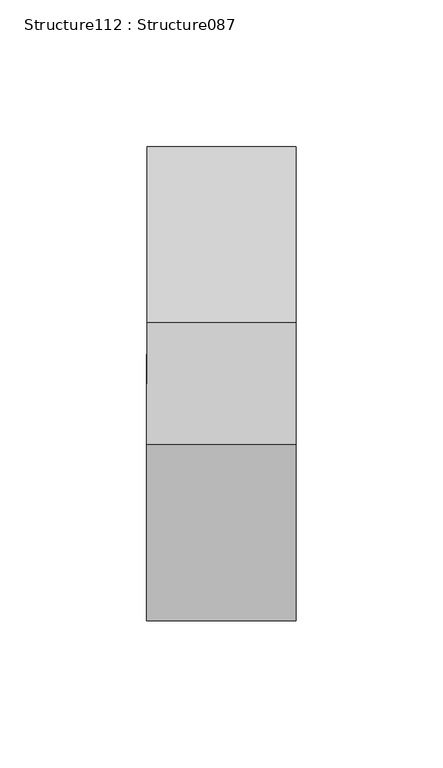
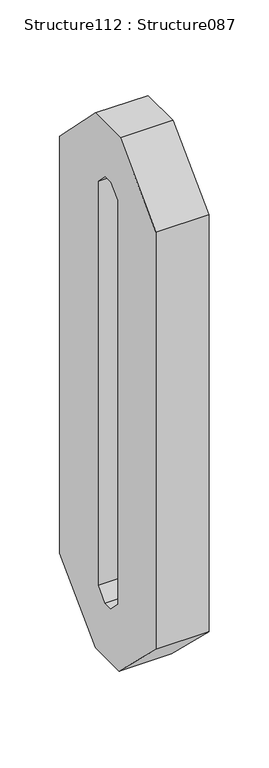
"""IFC4 building model written with IfcOpenShell, lengths in millimetres: proxy geometry, Structure112 : Structure087."""

import ifcopenshell
import ifcopenshell.guid

model = None  # the IFC model being written
_history = None  # IfcOwnerHistory: only IFC2X3 demands one
_inside = {}  # id of a spatial element -> (the spatial element, [elements in it])
_under = {}  # id of a project, library or spatial element -> (it, [spatial elements below it])
_declared = {}  # id of a project -> (the project, [libraries it declares])
_typed = {}  # id of a type object -> (the type object, [elements of that type])
_made_of = {}  # id of a material, layer set ... -> (it, [elements and type objects made of it])


def new_model(schema):
    """Start an empty IFC model of exactly this schema.

    Asked for "IFC4X3", IfcOpenShell would pick the latest addendum, in which some entities
    have other attributes; the version numbers below select the first issue.
    IFC2X3 requires an IfcOwnerHistory on every rooted entity: one is made here for all.
    """
    global model, _history
    if schema == "IFC4X3":
        model = ifcopenshell.file(schema_version=(4, 3, 0, 0))
    else:
        model = ifcopenshell.file(schema=schema)
    _inside.clear()
    _under.clear()
    _declared.clear()
    _typed.clear()
    _made_of.clear()
    _history = None
    if model.schema == "IFC2X3":
        org = make("IfcOrganization", Name="unknown")
        user = make(
            "IfcPersonAndOrganization",
            ThePerson=make("IfcPerson", FamilyName="unknown"),
            TheOrganization=org,
        )
        app = make(
            "IfcApplication",
            ApplicationDeveloper=org,
            Version="unknown",
            ApplicationFullName="unknown",
            ApplicationIdentifier="unknown",
        )
        _history = make(
            "IfcOwnerHistory",
            OwningUser=user,
            OwningApplication=app,
            ChangeAction="ADDED",
            CreationDate=0,
        )
    return model


def make(cls, **values):
    """One entity of the class cls with the attributes given. An attribute that is None is left unset."""
    return model.create_entity(
        cls, **{name: value for name, value in values.items() if value is not None}
    )


def rooted(cls, **values):
    """An entity with a GlobalId (a new one), such as an element, a storey or a relation."""
    return make(cls, GlobalId=ifcopenshell.guid.new(), OwnerHistory=_history, **values)


def si_unit(unit_type, name, prefix=None):
    """IfcSIUnit, for example si_unit("LENGTHUNIT", "METRE", prefix="MILLI")."""
    return make("IfcSIUnit", UnitType=unit_type, Prefix=prefix, Name=name)


def assignment(units):
    """IfcUnitAssignment: the units of a project."""
    return None if units is None else make("IfcUnitAssignment", Units=units)


def point(xyz):
    """IfcCartesianPoint."""
    return None if xyz is None else make("IfcCartesianPoint", Coordinates=xyz)


def direction(xyz):
    """IfcDirection."""
    return None if xyz is None else make("IfcDirection", DirectionRatios=xyz)


def frame(location, z_axis=None, x_axis=None):
    """IfcAxis2Placement3D, a coordinate frame: its origin and axes. An axis left out is left unset."""
    return make(
        "IfcAxis2Placement3D",
        Location=point(location),
        Axis=direction(z_axis),
        RefDirection=direction(x_axis),
    )


def origin():
    """The frame at (0, 0, 0) with its axes left unset."""
    return frame((0.0, 0.0, 0.0))


def place(relative_to, where):
    """IfcLocalPlacement: puts the frame where relative to a parent placement (None: the world)."""
    return make(
        "IfcLocalPlacement", PlacementRelTo=relative_to, RelativePlacement=where
    )


def context(
    kind, dimensions, precision=None, world=None, true_north=None, identifier=None
):
    """IfcGeometricRepresentationContext, for example the 3D "Model" context."""
    return make(
        "IfcGeometricRepresentationContext",
        ContextIdentifier=identifier,
        ContextType=kind,
        CoordinateSpaceDimension=dimensions,
        Precision=precision,
        WorldCoordinateSystem=world,
        TrueNorth=true_north,
    )


def project(units=None, contexts=None):
    """IfcProject with its units and contexts."""
    return rooted(
        "IfcProject",
        Name="project",
        RepresentationContexts=contexts,
        UnitsInContext=assignment(units),
    )


def spatial(cls, under=None, at=None, **own):
    """A site, building, storey or space (cls), placed at a placement, below another one or the project."""
    s = rooted(cls, ObjectPlacement=at, **own)
    if under is not None:
        _under.setdefault(under.id(), (under, []))[1].append(s)
    return s


def polyline(points):
    """IfcPolyline through the points."""
    return make("IfcPolyline", Points=[point(p) for p in points])


def outline(outer, holes=None, kind="AREA"):
    """IfcArbitraryClosedProfileDef: a profile drawn as a closed curve; with holes, ...WithVoids."""
    if holes is None:
        return make("IfcArbitraryClosedProfileDef", ProfileType=kind, OuterCurve=outer)
    return make(
        "IfcArbitraryProfileDefWithVoids",
        ProfileType=kind,
        OuterCurve=outer,
        InnerCurves=holes,
    )


def extrude(swept, where, along, depth):
    """IfcExtrudedAreaSolid: the profile swept, set in the frame where, extruded along a direction by depth."""
    return make(
        "IfcExtrudedAreaSolid",
        SweptArea=swept,
        Position=where,
        ExtrudedDirection=direction(along),
        Depth=depth,
    )


def shape(context_of_items, identifier, shape_type, items):
    """IfcShapeRepresentation: the items that make up one representation, for example the "Body"."""
    return make(
        "IfcShapeRepresentation",
        ContextOfItems=context_of_items,
        RepresentationIdentifier=identifier,
        RepresentationType=shape_type,
        Items=items,
    )


def source(mapping_origin, context_of_items, identifier, shape_type, items):
    """IfcRepresentationMap: a shape defined once, which mapped items show again and again."""
    return make(
        "IfcRepresentationMap",
        MappingOrigin=mapping_origin,
        MappedRepresentation=shape(context_of_items, identifier, shape_type, items),
    )


def transform(
    local_origin,
    x_axis=None,
    y_axis=None,
    z_axis=None,
    scale=None,
    scale2=None,
    scale3=None,
    uniform=True,
):
    """IfcCartesianTransformationOperator3D, or its non-uniform kind. x_axis, y_axis, z_axis: its Axis1, 2, 3."""
    if uniform:
        return make(
            "IfcCartesianTransformationOperator3D",
            Axis1=direction(x_axis),
            Axis2=direction(y_axis),
            LocalOrigin=point(local_origin),
            Scale=scale,
            Axis3=direction(z_axis),
        )
    return make(
        "IfcCartesianTransformationOperator3DnonUniform",
        Axis1=direction(x_axis),
        Axis2=direction(y_axis),
        LocalOrigin=point(local_origin),
        Scale=scale,
        Axis3=direction(z_axis),
        Scale2=scale2,
        Scale3=scale3,
    )


def mapped(mapping_source, mapping_target):
    """IfcMappedItem: shows the shape of a source again, moved by a transform."""
    return make(
        "IfcMappedItem", MappingSource=mapping_source, MappingTarget=mapping_target
    )


def made_of(thing, what):
    """Note that an element or type object is made of a material, layer set ...; save() writes the relation."""
    if what is not None:
        _made_of.setdefault(what.id(), (what, []))[1].append(thing)
    return thing


def element(
    cls,
    number,
    at=None,
    inside=None,
    cuts=None,
    type_object=None,
    material=None,
    context=None,
    identifier="Body",
    shape_type=None,
    held_by="IfcProductDefinitionShape",
    body=None,
    shapes=None,
    **own,
):
    """One element of the class cls, such as IfcWall. Its Tag is "e" and its number.

    at: its placement. inside: the storey or other place that contains it. cuts: it is an
    opening in that element (IfcRelVoidsElement). A single representation is given by context,
    identifier, shape_type and body (its items); several are given by shapes. held_by: the class
    of the entity that holds the representations. save() writes the other relations.
    """
    e = rooted(cls, Tag="e%d" % number, ObjectPlacement=at, **own)
    if body is not None:
        shapes = [shape(context, identifier, shape_type, body)]
    if shapes is not None:
        e.Representation = make(held_by, Representations=shapes)
    if inside is not None:
        _inside.setdefault(inside.id(), (inside, []))[1].append(e)
    if cuts is not None:
        rooted(
            "IfcRelVoidsElement", RelatingBuildingElement=cuts, RelatedOpeningElement=e
        )
    if type_object is not None:
        _typed.setdefault(type_object.id(), (type_object, []))[1].append(e)
    return made_of(e, material)


def aggregate(whole, parts):
    """IfcRelAggregates: a whole, such as a stair, and the parts it consists of."""
    return rooted("IfcRelAggregates", RelatingObject=whole, RelatedObjects=parts)


def save(model, path):
    """Write the relations noted so far, then the file.

    IfcRelAggregates (storeys below a building ...), IfcRelContainedInSpatialStructure (elements
    in a storey), IfcRelDefinesByType, IfcRelAssociatesMaterial and IfcRelDeclares: one each for
    every whole, place, type object, material and project.
    """
    for whole, parts in _under.values():
        aggregate(whole, parts)
    for where, things in _inside.values():
        rooted(
            "IfcRelContainedInSpatialStructure",
            RelatedElements=things,
            RelatingStructure=where,
        )
    for kind, things in _typed.values():
        rooted("IfcRelDefinesByType", RelatedObjects=things, RelatingType=kind)
    for what, things in _made_of.values():
        rooted("IfcRelAssociatesMaterial", RelatedObjects=things, RelatingMaterial=what)
    for by, libraries in _declared.values():
        rooted("IfcRelDeclares", RelatingContext=by, RelatedDefinitions=libraries)
    model.write(path)


def structure112_structure087_d23aebd8(model_context):
    return source(origin(), model_context, "Body", "SweptSolid", [
        extrude(outline(polyline([(425.6202752, 0.0), (485.5454951, -59.9250696), (485.5454951, -101.4135448), (425.6204255, -161.3386144), (-0.0006857, -161.3379027), (-59.8837361, -99.1882102), (-59.9250696, -59.9250696), (0.0, 0.0), (425.6202752, 0.0)]), holes=[polyline([(-4.610305, -85.2790784), (6.9144584, -96.8039514), (418.7015877, -96.8039514), (430.2261049, -85.2794342), (430.2261049, -76.0616707), (418.7015877, -64.5371537), (6.9145779, -64.5371537), (-4.6099492, -76.0616707), (-4.610305, -85.2790784)])]), frame((-56111.1155572, 292138.2469641, -109.9449396), z_axis=(-0.9999998917542984, 0.00046528635450596156, 0.0), x_axis=(0.0, 0.0, 1.0)), (0.0, 0.0, 1.0), 50.8),
    ])


if __name__ == "__main__":
    model = new_model("IFC4")
    model_context = context("Model", 3, world=origin())
    ifc_project = project(units=[si_unit("LENGTHUNIT", "METRE", prefix="MILLI")], contexts=[model_context])
    site = spatial("IfcSite", under=ifc_project)
    building = spatial("IfcBuilding", under=site)
    placement = place(None, origin())
    structure112_structure087_shape = structure112_structure087_d23aebd8(model_context)
    element("IfcBuildingElementProxy", 1, Name="Structure112 : Structure087", ObjectType="Structure112 : Structure087", at=placement, inside=building, context=model_context, shape_type="MappedRepresentation", body=[
        mapped(structure112_structure087_shape, transform((0.0, 0.0, 0.0), x_axis=(1.0, 0.0, 0.0), y_axis=(0.0, 1.0, 0.0), z_axis=(0.0, 0.0, 1.0))),
    ])
    save(model, "model.ifc")

# Revit data of these elements
# Type "Structure112 : Structure087"
#   NameOverride = "Structure087"
# Element 1 (IfcBuildingElementProxy, "Structure112 : Structure087")
#   Materials on its faces: "BRUSHED ALUMINUM LETTERING"
# Materials
#   "BRUSHED ALUMINUM LETTERING": class "Unassigned", colour RGB 169 181 186, transparency 0, Cost = 0
